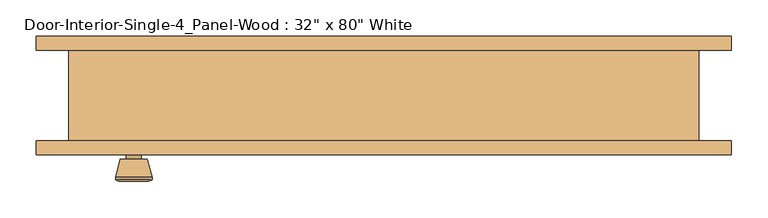
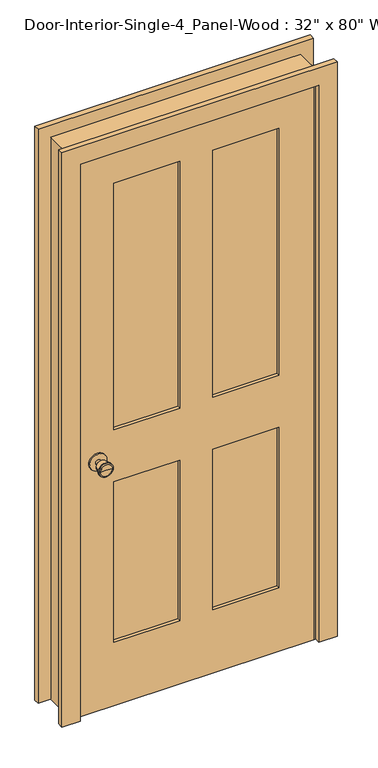
"""IFC4 building model written with IfcOpenShell, lengths in millimetres: door geometry."""

from ifc_helpers import new_model, si_unit, point, frame, frame_2d, origin, place, context, project, spatial, polyline, circle_curve, trimmed, segment, composite_curve, outline, extrude, faceted_brep, source, transform, mapped, element, save
from ifc_brep_helpers import plane_surface, cylinder_surface, revolved_surface, advanced_brep


def door_4e624a36(model_context):
    return source(origin(), model_context, "Body", "SolidModel", [
        advanced_brep(
        [(-342.9, -17.8125, 914.4), (-352.9, -17.8125, 914.4), (-332.9, -17.8125, 914.4), (-322.4241324, 31.1875, 914.4), (-363.3758676, 31.1875, 914.4), (-342.9, 31.1875, 914.4), (-317.9, 29.3596319, 914.4), (-367.9, 29.3596319, 914.4), (-317.9, 25.8959537, 914.4), (-367.9, 25.8959537, 914.4), (-324.263764, 1.1875, 914.4), (-361.536236, 1.1875, 914.4), (-332.9, 1.1875, 914.4), (-352.9, 1.1875, 914.4)],
        [
            (0, 1),
            (1, 2, circle_curve(frame((-342.9, -17.8125, 914.4), z_axis=(0.0, -1.0, 0.0), x_axis=(-1.0, 0.0, 0.0)), 10.0)),
            (2, 0),
            (2, 1, circle_curve(frame((-342.9, -17.8125, 914.4), z_axis=(0.0, -1.0, 0.0), x_axis=(-1.0, 0.0, 0.0)), 10.0)),
            (3, 4, circle_curve(frame((-342.9, 31.1875, 914.4), z_axis=(0.0, 1.0, 0.0), x_axis=(-1.0, 0.0, 0.0)), 20.4758676)),
            (4, 5),
            (5, 3),
            (4, 3, circle_curve(frame((-342.9, 31.1875, 914.4), z_axis=(0.0, 1.0, 0.0), x_axis=(-1.0, 0.0, 0.0)), 20.4758676)),
            (6, 7, circle_curve(frame((-342.9, 29.3596319, 914.4), z_axis=(0.0, 1.0, 0.0), x_axis=(-1.0, 0.0, 0.0)), 25.0)),
            (7, 4),
            (3, 6),
            (7, 6, circle_curve(frame((-342.9, 29.3596319, 914.4), z_axis=(0.0, 1.0, 0.0), x_axis=(-1.0, 0.0, 0.0)), 25.0)),
            (8, 9, circle_curve(frame((-342.9, 25.8959537, 914.4), z_axis=(0.0, 1.0, 0.0), x_axis=(-1.0, 0.0, 0.0)), 25.0)),
            (9, 7),
            (6, 8),
            (9, 8, circle_curve(frame((-342.9, 25.8959537, 914.4), z_axis=(0.0, 1.0, 0.0), x_axis=(-1.0, 0.0, 0.0)), 25.0)),
            (10, 11, circle_curve(frame((-342.9, 1.1875, 914.4), z_axis=(0.0, 1.0, 0.0), x_axis=(-1.0, 0.0, 0.0)), 18.636236)),
            (11, 9),
            (8, 10),
            (11, 10, circle_curve(frame((-342.9, 1.1875, 914.4), z_axis=(0.0, 1.0, 0.0), x_axis=(-1.0, 0.0, 0.0)), 18.636236)),
            (12, 13, circle_curve(frame((-342.9, 1.1875, 914.4), z_axis=(0.0, 1.0, 0.0), x_axis=(-1.0, 0.0, 0.0)), 10.0)),
            (13, 11),
            (10, 12),
            (13, 12, circle_curve(frame((-342.9, 1.1875, 914.4), z_axis=(0.0, 1.0, 0.0), x_axis=(-1.0, 0.0, 0.0)), 10.0)),
            (1, 13),
            (12, 2),
        ],
        [
            plane_surface(frame((-342.9, -17.8125, 914.4), z_axis=(0.0, -1.0, 0.0), x_axis=(-1.0, 0.0, 0.0))),
            plane_surface(frame((-342.9, 31.1875, 914.4), z_axis=(0.0, 1.0, 0.0), x_axis=(-1.0, 0.0, 0.0))),
            revolved_surface(polyline([(-363.3758676, 31.1875, 914.4), (-367.9, 29.3596319, 914.4)]), (-342.9, -17.8125, 914.4), (0.0, -1.0, 0.0)),
            cylinder_surface(frame((-342.9, -17.8125, 914.4), z_axis=(0.0, -1.0, 0.0), x_axis=(-1.0, 0.0, 0.0)), 25.0),
            revolved_surface(polyline([(-367.9, 25.8959537, 914.4), (-361.536236, 1.1875, 914.4)]), (-342.9, -17.8125, 914.4), (0.0, -1.0, 0.0)),
            plane_surface(frame((-342.9, 1.1875, 914.4), z_axis=(0.0, -1.0, 0.0), x_axis=(-1.0, 0.0, 0.0))),
            cylinder_surface(frame((-342.9, -17.8125, 914.4), z_axis=(0.0, -1.0, 0.0), x_axis=(-1.0, 0.0, 0.0)), 10.0),
        ],
        [
            (0, [[1, 2, 3]]),
            (0, [[-3, 4, -1]]),
            (1, [[5, 6, 7]]),
            (1, [[8, -7, -6]]),
            (2, [[9, 10, -5, 11]]),
            (2, [[12, -11, -8, -10]]),
            (3, [[13, 14, -9, 15]]),
            (3, [[16, -15, -12, -14]]),
            (4, [[17, 18, -13, 19]]),
            (4, [[20, -19, -16, -18]]),
            (5, [[21, 22, -17, 23]]),
            (5, [[24, -23, -20, -22]]),
            (6, [[-2, 25, -21, 26]]),
            (6, [[-4, -26, -24, -25]]),
        ],
    ),
        extrude(outline(composite_curve([segment(trimmed(circle_curve(frame_2d((914.4, -342.9)), 30.0), [point((914.4, -372.9))], [point((914.4, -312.9))], False, "CARTESIAN"), True, "CONTINUOUS"), segment(trimmed(circle_curve(frame_2d((914.4, -342.9)), 30.0), [point((914.4, -312.9))], [point((914.4, -372.9))], False, "CARTESIAN"), True, "CONTINUOUS")], self_intersect=False)), frame((0.0, -23.8125, 0.0), z_axis=(0.0, 1.0, 0.0), x_axis=(0.0, 0.0, 1.0)), (0.0, 0.0, 1.0), 6.0),
        advanced_brep(
        [(-342.9, -64.7375, 914.4), (-332.9, -64.7375, 914.4), (-352.9, -64.7375, 914.4), (-322.4241324, -113.7375, 914.4), (-342.9, -113.7375, 914.4), (-363.3758676, -113.7375, 914.4), (-317.9, -111.9096319, 914.4), (-367.9, -111.9096319, 914.4), (-317.9, -108.4459537, 914.4), (-367.9, -108.4459537, 914.4), (-324.263764, -83.7375, 914.4), (-361.536236, -83.7375, 914.4), (-332.9, -83.7375, 914.4), (-352.9, -83.7375, 914.4)],
        [
            (0, 1),
            (1, 2, circle_curve(frame((-342.9, -64.7375, 914.4), z_axis=(0.0, 1.0, 0.0), x_axis=(-1.0, 0.0, 0.0)), 10.0)),
            (2, 0),
            (2, 1, circle_curve(frame((-342.9, -64.7375, 914.4), z_axis=(0.0, 1.0, 0.0), x_axis=(-1.0, 0.0, 0.0)), 10.0)),
            (3, 4),
            (4, 5),
            (5, 3, circle_curve(frame((-342.9, -113.7375, 914.4), z_axis=(0.0, -1.0, 0.0), x_axis=(-1.0, 0.0, 0.0)), 20.4758676)),
            (3, 5, circle_curve(frame((-342.9, -113.7375, 914.4), z_axis=(0.0, -1.0, 0.0), x_axis=(-1.0, 0.0, 0.0)), 20.4758676)),
            (6, 3),
            (5, 7),
            (7, 6, circle_curve(frame((-342.9, -111.9096319, 914.4), z_axis=(0.0, -1.0, 0.0), x_axis=(-1.0, 0.0, 0.0)), 25.0)),
            (6, 7, circle_curve(frame((-342.9, -111.9096319, 914.4), z_axis=(0.0, -1.0, 0.0), x_axis=(-1.0, 0.0, 0.0)), 25.0)),
            (8, 6),
            (7, 9),
            (9, 8, circle_curve(frame((-342.9, -108.4459537, 914.4), z_axis=(0.0, -1.0, 0.0), x_axis=(-1.0, 0.0, 0.0)), 25.0)),
            (8, 9, circle_curve(frame((-342.9, -108.4459537, 914.4), z_axis=(0.0, -1.0, 0.0), x_axis=(-1.0, 0.0, 0.0)), 25.0)),
            (10, 8),
            (9, 11),
            (11, 10, circle_curve(frame((-342.9, -83.7375, 914.4), z_axis=(0.0, -1.0, 0.0), x_axis=(-1.0, 0.0, 0.0)), 18.636236)),
            (10, 11, circle_curve(frame((-342.9, -83.7375, 914.4), z_axis=(0.0, -1.0, 0.0), x_axis=(-1.0, 0.0, 0.0)), 18.636236)),
            (12, 10),
            (11, 13),
            (13, 12, circle_curve(frame((-342.9, -83.7375, 914.4), z_axis=(0.0, -1.0, 0.0), x_axis=(-1.0, 0.0, 0.0)), 10.0)),
            (12, 13, circle_curve(frame((-342.9, -83.7375, 914.4), z_axis=(0.0, -1.0, 0.0), x_axis=(-1.0, 0.0, 0.0)), 10.0)),
            (1, 12),
            (13, 2),
        ],
        [
            plane_surface(frame((-342.9, -64.7375, 914.4), z_axis=(0.0, 1.0, 0.0), x_axis=(-1.0, 0.0, 0.0))),
            plane_surface(frame((-342.9, -113.7375, 914.4), z_axis=(0.0, -1.0, 0.0), x_axis=(-1.0, 0.0, 0.0))),
            revolved_surface(polyline([(-363.3758676, -113.7375, 914.4), (-367.9, -111.9096319, 914.4)]), (-342.9, -64.7375, 914.4), (0.0, 1.0, 0.0)),
            cylinder_surface(frame((-342.9, -64.7375, 914.4), z_axis=(0.0, 1.0, 0.0), x_axis=(-1.0, 0.0, 0.0)), 25.0),
            revolved_surface(polyline([(-367.9, -108.4459537, 914.4), (-361.536236, -83.7375, 914.4)]), (-342.9, -64.7375, 914.4), (0.0, 1.0, 0.0)),
            plane_surface(frame((-342.9, -83.7375, 914.4), z_axis=(0.0, 1.0, 0.0), x_axis=(-1.0, 0.0, 0.0))),
            cylinder_surface(frame((-342.9, -64.7375, 914.4), z_axis=(0.0, 1.0, 0.0), x_axis=(-1.0, 0.0, 0.0)), 10.0),
        ],
        [
            (0, [[1, 2, 3]]),
            (0, [[-3, 4, -1]]),
            (1, [[5, 6, 7]]),
            (1, [[-6, -5, 8]]),
            (2, [[9, -7, 10, 11]]),
            (2, [[-10, -8, -9, 12]]),
            (3, [[13, -11, 14, 15]]),
            (3, [[-14, -12, -13, 16]]),
            (4, [[17, -15, 18, 19]]),
            (4, [[-18, -16, -17, 20]]),
            (5, [[21, -19, 22, 23]]),
            (5, [[-22, -20, -21, 24]]),
            (6, [[25, -23, 26, -2]]),
            (6, [[-26, -24, -25, -4]]),
        ],
    ),
        extrude(outline(composite_curve([segment(trimmed(circle_curve(frame_2d((914.4, -342.9)), 30.0), [point((914.4, -372.9))], [point((914.4, -312.9))], False, "CARTESIAN"), True, "CONTINUOUS"), segment(trimmed(circle_curve(frame_2d((914.4, -342.9)), 30.0), [point((914.4, -312.9))], [point((914.4, -372.9))], False, "CARTESIAN"), True, "CONTINUOUS")], self_intersect=False)), frame((0.0, -64.7375, 0.0), z_axis=(0.0, 1.0, 0.0), x_axis=(0.0, 0.0, 1.0)), (0.0, 0.0, 1.0), 6.0),
        extrude(outline(polyline([(285.75, -35.4541667), (285.75, -47.0958333), (57.15, -47.0958333), (57.15, -35.4541667), (285.75, -35.4541667)])), frame((0.0, 0.0, 1009.65), z_axis=(0.0, 0.0, 1.0), x_axis=(1.0, 0.0, 0.0)), (0.0, 0.0, 1.0), 903.2875),
        extrude(outline(polyline([(-57.15, -35.4541667), (-57.15, -47.0958333), (-285.75, -47.0958333), (-285.75, -35.4541667), (-57.15, -35.4541667)])), frame((0.0, 0.0, 1009.65), z_axis=(0.0, 0.0, 1.0), x_axis=(1.0, 0.0, 0.0)), (0.0, 0.0, 1.0), 903.2875),
        extrude(outline(polyline([(285.75, -35.4541667), (285.75, -47.0958333), (57.15, -47.0958333), (57.15, -35.4541667), (285.75, -35.4541667)])), frame((0.0, 0.0, 231.775), z_axis=(0.0, 0.0, 1.0), x_axis=(1.0, 0.0, 0.0)), (0.0, 0.0, 1.0), 587.375),
        extrude(outline(polyline([(-57.15, -35.4541667), (-57.15, -47.0958333), (-285.75, -47.0958333), (-285.75, -35.4541667), (-57.15, -35.4541667)])), frame((0.0, 0.0, 231.775), z_axis=(0.0, 0.0, 1.0), x_axis=(1.0, 0.0, 0.0)), (0.0, 0.0, 1.0), 587.375),
        extrude(outline(polyline([(2032.0, -406.4), (0.0, -406.4), (0.0, 406.4), (2032.0, 406.4), (2032.0, -406.4)]), holes=[polyline([(1912.9375, 57.15), (1912.9375, 285.75), (1009.65, 285.75), (1009.65, 57.15), (1912.9375, 57.15)]), polyline([(1009.65, -57.15), (1009.65, -285.75), (1912.9375, -285.75), (1912.9375, -57.15), (1009.65, -57.15)]), polyline([(819.15, 57.15), (819.15, 285.75), (231.775, 285.75), (231.775, 57.15), (819.15, 57.15)]), polyline([(231.775, -57.15), (231.775, -285.75), (819.15, -285.75), (819.15, -57.15), (231.775, -57.15)])]), frame((0.0, -58.7375, 0.0), z_axis=(0.0, 1.0, 0.0), x_axis=(0.0, 0.0, 1.0)), (0.0, 0.0, 1.0), 34.925),
        faceted_brep([(431.8, -58.7375, 0.0), (406.4, -58.7375, 0.0), (406.4, -23.8125, 0.0), (393.7, -23.8125, 0.0), (393.7, 11.1125, 0.0), (406.4, 11.1125, 0.0), (406.4, 65.0875, 0.0), (431.8, 65.0875, 0.0), (431.8, 65.0875, 2057.4), (431.8, -58.7375, 2057.4), (406.4, 65.0875, 2032.0), (-406.4, 65.0875, 2032.0), (-406.4, 65.0875, 0.0), (-431.8, 65.0875, 0.0), (-431.8, 65.0875, 2057.4), (406.4, 11.1125, 2032.0), (393.7, 11.1125, 2019.3), (-393.7, 11.1125, 2019.3), (-393.7, 11.1125, 0.0), (-406.4, 11.1125, 0.0), (-406.4, 11.1125, 2032.0), (393.7, -23.8125, 2019.3), (406.4, -23.8125, 2032.0), (-406.4, -23.8125, 2032.0), (-406.4, -23.8125, 0.0), (-393.7, -23.8125, 0.0), (-393.7, -23.8125, 2019.3), (406.4, -58.7375, 2032.0), (-431.8, -58.7375, 2057.4), (-431.8, -58.7375, 0.0), (-406.4, -58.7375, 0.0), (-406.4, -58.7375, 2032.0)], [[[0, 1, 2, 3, 4, 5, 6, 7]], [[7, 8, 9, 0]], [[6, 10, 11, 12, 13, 14, 8, 7]], [[5, 15, 10, 6]], [[4, 16, 17, 18, 19, 20, 15, 5]], [[3, 21, 16, 4]], [[2, 22, 23, 24, 25, 26, 21, 3]], [[1, 27, 22, 2]], [[0, 9, 28, 29, 30, 31, 27, 1]], [[8, 14, 28, 9]], [[15, 20, 11, 10]], [[21, 26, 17, 16]], [[27, 31, 23, 22]], [[29, 13, 12, 19, 18, 25, 24, 30]], [[14, 13, 29, 28]], [[20, 19, 12, 11]], [[26, 25, 18, 17]], [[31, 30, 24, 23]]]),
        extrude(outline(polyline([(0.0, 476.25), (2101.85, 476.25), (2101.85, -476.25), (0.0, -476.25), (0.0, -412.75), (2038.35, -412.75), (2038.35, 412.75), (0.0, 412.75), (0.0, 476.25)])), frame((0.0, 65.0875, 0.0), z_axis=(0.0, 1.0, 0.0), x_axis=(0.0, 0.0, 1.0)), (0.0, 0.0, 1.0), 19.05),
        extrude(outline(polyline([(0.0, 476.25), (2101.85, 476.25), (2101.85, -476.25), (0.0, -476.25), (0.0, -412.75), (2038.35, -412.75), (2038.35, 412.75), (0.0, 412.75), (0.0, 476.25)])), frame((0.0, -77.7875, 0.0), z_axis=(0.0, 1.0, 0.0), x_axis=(0.0, 0.0, 1.0)), (0.0, 0.0, 1.0), 19.05),
    ])


if __name__ == "__main__":
    model = new_model("IFC4")
    model_context = context("Model", 3, world=origin())
    ifc_project = project(units=[si_unit("LENGTHUNIT", "METRE", prefix="MILLI")], contexts=[model_context])
    site = spatial("IfcSite", under=ifc_project)
    building = spatial("IfcBuilding", under=site)
    placement = place(None, origin())
    door_shape = door_4e624a36(model_context)
    element("IfcDoor", 1, ObjectType="Door-Interior-Single-4_Panel-Wood : 32\" x 80\" White", at=placement, inside=building, context=model_context, shape_type="MappedRepresentation", body=[
        mapped(door_shape, transform((0.0, 0.0, 0.0), x_axis=(1.0, 0.0, 0.0), y_axis=(0.0, 1.0, 0.0), z_axis=(0.0, 0.0, 1.0))),
    ])
    save(model, "model.ifc")

# Revit data of these elements
# Type "Door-Interior-Single-4_Panel-Wood : 32\" x 80\" White"
#   Type Mark = "48"
#   COBie.Type.CreatedBy = "doug.wood@us.ibm.com"
#   COBie.Type.CreatedOn = "2016-04-14T02:07:24"
#   COBie.Type.Name = "Doors_Door-Interior-Single-4_Panel-Wood_32\" x 80\" White_48"
#   COBie.Type.Category = "23-30 10 00 : Doors"
#   COBie.Type.Description = "Door-Interior-Single-4_Panel-Wood_32\" x 80\" White"
#   COBie.Type.Manufacturer = ""
#   COBie.Type.ModelNumber = ""
#   Assembly Code = "C1020300"
#   Analytic Construction = "Wooden"
#   COBie.Type.ReplacementCost = 0
#   Top Rail = 0' - 4 11/16"
#   Thickness = 0' - 1 3/8"
#   Thermal Resistance (R) = 0.455703 (m²·K)/W
#   Swing Angle [instance default] = 90.00°
#   Stiles = 0' - 4 3/4"
#   Rough Width = 2' - 10"
#   Rough Height = 6' - 9"
#   Mullion = 0' - 4 1/2"
#   Lock Rail = 0' - 7 1/2"
#   Height = 6' - 8"
#   Width = 2' - 8"
#   Heat Transfer Coefficient (U) = 2.19465 W/(m²·K)
#   Bottom Rail = 0' - 9 1/8"
#   COBie.Type = no
#   Trim Material = Trim - White
#   Panel Material = Door - Panel - White
#   Frame Material = Door - Panel - White
#   Door Handle Material = ARCAT - Metal - Brass, Polished
#   Visual Light Transmittance = 0
#   Solar Heat Gain Coefficient = 0
#   Wall Closure = (empty or 0)
#   Function = (empty or 0)
# Element 1 (IfcDoor, "Door-Interior-Single-4_Panel-Wood : 32\" x 80\" White")
#   Materials on its faces: "Door - Panel - White", "ARCAT - Metal - Brass, Polished", "Trim - White"
# Materials
#   "Trim - White": class "Wood", colour RGB 255 255 255, transparency 0, Cost = 0
#   "Door - Panel - White": class "Wood", colour RGB 255 255 255, transparency 0, Cost = 0
#   "ARCAT - Metal - Brass, Polished": class "Unassigned", colour RGB 246 240 166, transparency 0, Keynote = "05050", Model = "Generic", Manufacturer = "Generic", Description = "Steel, Chrome Plated"
